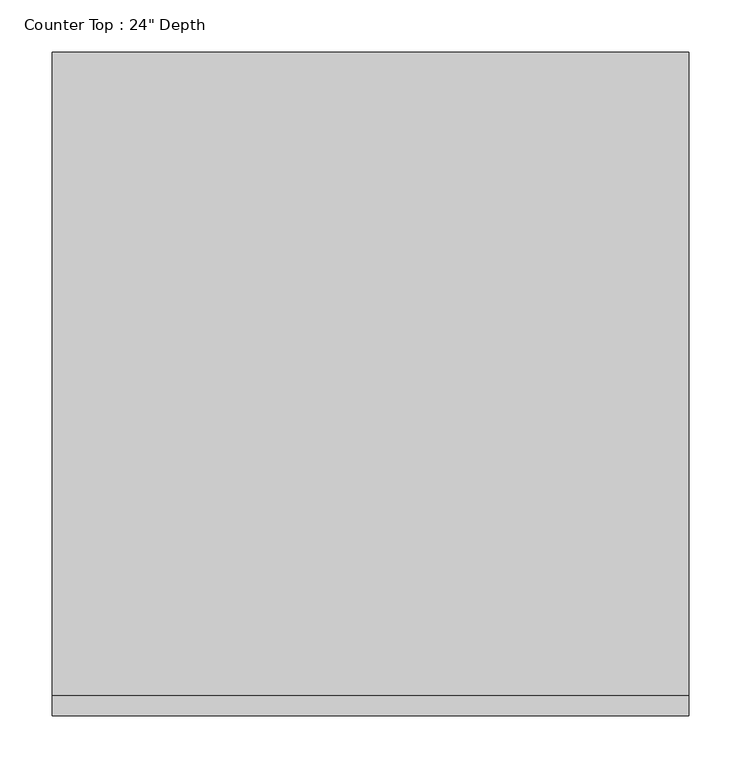
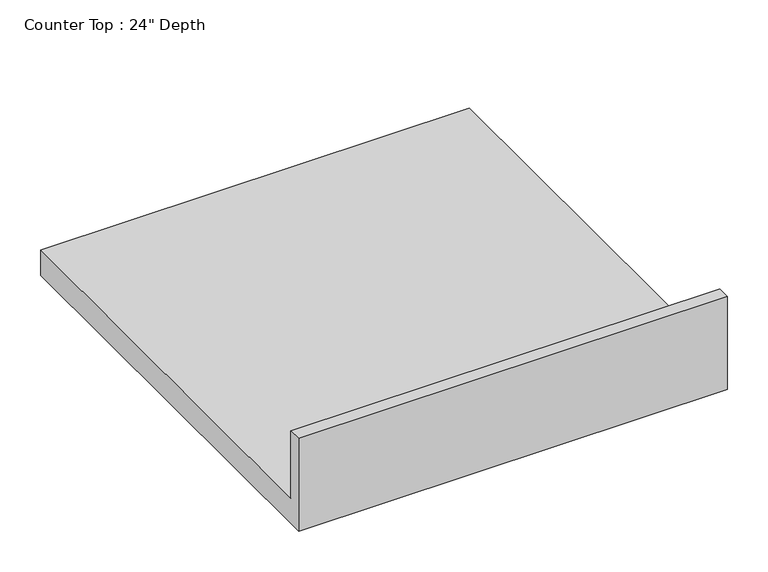
"""IFC4 building model written with IfcOpenShell, lengths in millimetres: furniture geometry."""

from ifc_helpers import new_model, si_unit, frame, origin, place, context, project, spatial, polyline, outline, extrude, source, transform, mapped, element, save


def furniture_c90ff350(model_context):
    return source(origin(), model_context, "Body", "SweptSolid", [
        extrude(outline(polyline([(0.0, 1016.0), (19.05, 1016.0), (19.05, 914.4), (635.0, 914.4), (635.0, 876.3), (0.0, 876.3), (0.0, 1016.0)])), frame((-1200.4622951, 0.0, 0.0), z_axis=(1.0, 0.0, 0.0), x_axis=(0.0, 1.0, 0.0)), (0.0, 0.0, 1.0), 609.6),
    ])


if __name__ == "__main__":
    model = new_model("IFC4")
    model_context = context("Model", 3, world=origin())
    ifc_project = project(units=[si_unit("LENGTHUNIT", "METRE", prefix="MILLI")], contexts=[model_context])
    site = spatial("IfcSite", under=ifc_project)
    building = spatial("IfcBuilding", under=site)
    placement = place(None, origin())
    furniture_shape = furniture_c90ff350(model_context)
    element("IfcFurniture", 1, ObjectType="Counter Top : 24\" Depth", at=placement, inside=building, context=model_context, shape_type="MappedRepresentation", body=[
        mapped(furniture_shape, transform((0.0, 0.0, 0.0), x_axis=(1.0, 0.0, 0.0), y_axis=(0.0, 1.0, 0.0), z_axis=(0.0, 0.0, 1.0))),
    ])
    save(model, "model.ifc")

# Revit data of these elements
# Type "Counter Top : 24\" Depth"
#   Assembly Code = "C1030400"
#   Counter Thickness = 0' - 1 1/2"
#   Depth = 2' - 1"
#   Height = 3' - 0"
#   Length [instance default] = 8' - 0"
#   Counter Top Material = Laminate, Blue, Matte
#   Default Elevation = 0
# Element 1 (IfcFurniture, "Counter Top : 24\" Depth")
#   Length = 2' - 0"
#   Materials on its faces: "Laminate, Blue, Matte"
# Materials
#   "Laminate, Blue, Matte": class "Plastic", colour RGB 85 101 155, transparency 0, Description = "Plastic Laminate - Blue, Matte", Cost = 0
